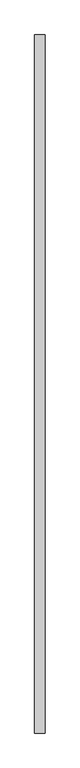
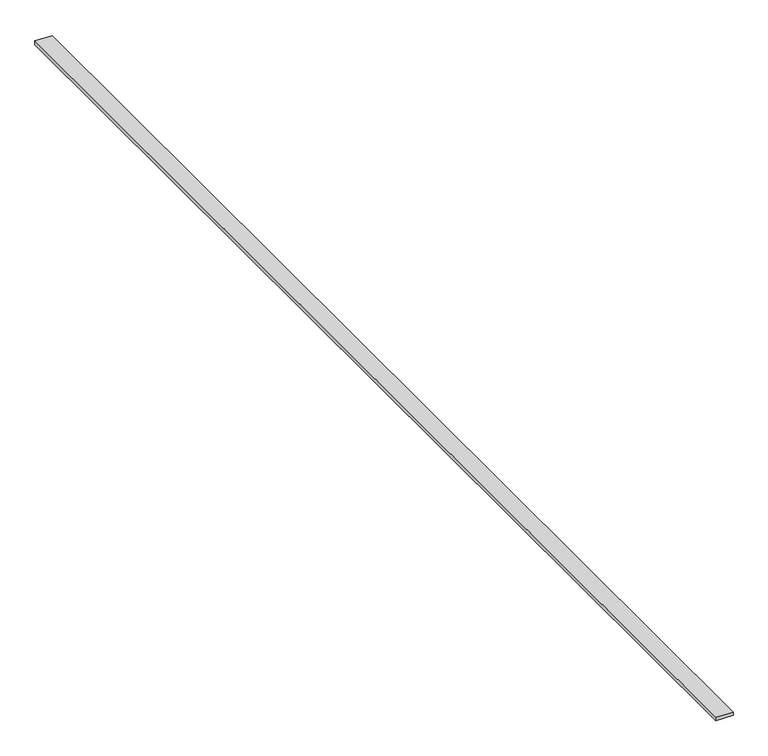
"""IFC4 building model written with IfcOpenShell, lengths in millimetres: proxy geometry, Generic Models 7:Generic Models 1:337419:Generic Models 1:337419 : Generic Models 7:Generic Models 1:337419:30 : Generic Models 7:Generic Models 1:337419:Generic Models 1:337419 : Generic Models 7:Generic Models 1:337419:301336."""

from ifc_helpers import new_model, si_unit, frame, origin, place, context, project, spatial, polyline, outline, extrude, source, transform, mapped, element, save


def generic_models_6fe2bc36(model_context):
    return source(origin(), model_context, "Body", "SweptSolid", [
        extrude(outline(polyline([(6135.290625, 560365.6617239), (6135.290625, 560549.8117239), (6169.4995614, 560549.8117239), (6179.1504539, 560365.6617239), (6135.290625, 560365.6617239)])), frame((0.0, -578946.7163842, 0.0), z_axis=(0.0, 1.0, 0.0), x_axis=(0.0, 0.0, 1.0)), (0.0, 0.0, 1.0), 12477.75),
    ])


if __name__ == "__main__":
    model = new_model("IFC4")
    model_context = context("Model", 3, world=origin())
    ifc_project = project(units=[si_unit("LENGTHUNIT", "METRE", prefix="MILLI")], contexts=[model_context])
    site = spatial("IfcSite", under=ifc_project)
    building = spatial("IfcBuilding", under=site)
    placement = place(None, origin())
    generic_models_shape = generic_models_6fe2bc36(model_context)
    element("IfcBuildingElementProxy", 1, Name="Generic Models 7:Generic Models 1:337419:Generic Models 1:337419 : Generic Models 7:Generic Models 1:337419:30 : Generic Models 7:Generic Models 1:337419:Generic Models 1:337419 : Generic Models 7:Generic Models 1:337419:301336", ObjectType="Generic Models 7:Generic Models 1:337419:Generic Models 1:337419 : Generic Models 7:Generic Models 1:337419:30 : Generic Models 7:Generic Models 1:337419:Generic Models 1:337419 : Generic Models 7:Generic Models 1:337419:301336", at=placement, inside=building, context=model_context, shape_type="MappedRepresentation", body=[
        mapped(generic_models_shape, transform((0.0, 0.0, 0.0), x_axis=(1.0, 0.0, 0.0), y_axis=(0.0, 1.0, 0.0), z_axis=(0.0, 0.0, 1.0))),
    ])
    save(model, "model.ifc")

# Revit data of these elements
# Type "Generic Models 7:Generic Models 1:337419:Generic Models 1:337419 : Generic Models 7:Generic Models 1:337419:30 : Generic Models 7:Generic Models 1:337419:Generic Models 1:337419 : Generic Models 7:Generic Models 1:337419:301336"
#   NameOverride = "Generic Models 7:Generic Models 1:337419:Generic Models 1:337419 : Generic Models 7:Generic Models 1:337419:301336"
#   ObjectTypeOverride = "Generic Models 1:337419 : Generic Models 7:Generic Models 1:337419"
#   Reference = "Generic Models 1"
#   Tag = "301336"
# Element 1 (IfcBuildingElementProxy, "Generic Models 7:Generic Models 1:337419:Generic Models 1:337419 : Generic Models 7:Generic Models 1:337419:30 : Generic Models 7:Generic Models 1:337419:Generic Models 1:337419 : Generic Models 7:Generic Models 1:337419:301336")
#   Materials on its faces: "WOOD BLOCKING - SIZE AS NECESSARY"
# Materials
#   "WOOD BLOCKING - SIZE AS NECESSARY": class "Wood", colour RGB 144 113 62, transparency 0, Description = "Pinus Echinata", Cost = 0
